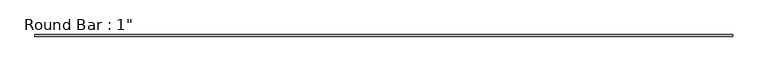
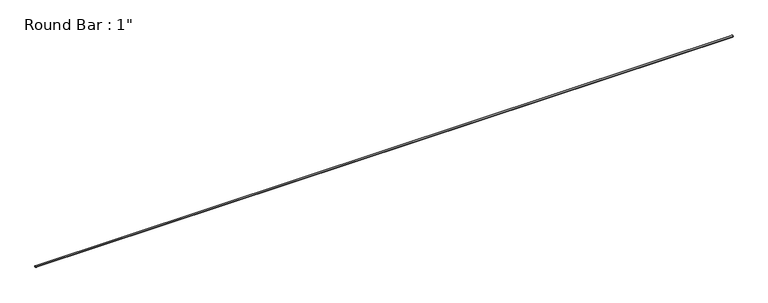
"""IFC4 building model written with IfcOpenShell, lengths in millimetres: member geometry."""

from ifc_helpers import new_model, si_unit, point, frame, origin, origin_2d, place, context, project, spatial, circle_curve, trimmed, segment, composite_curve, outline, extrude, source, transform, mapped, element, save


def member_a7b351ab(model_context):
    return source(origin(), model_context, "Body", "SweptSolid", [
        extrude(outline(composite_curve([segment(trimmed(circle_curve(origin_2d(), 12.7), [point((-12.7, 0.0))], [point((12.7, 0.0))], False, "CARTESIAN"), True, "CONTINUOUS"), segment(trimmed(circle_curve(origin_2d(), 12.7), [point((12.7, 0.0))], [point((-12.7, 0.0))], False, "CARTESIAN"), True, "CONTINUOUS")], self_intersect=False)), frame((-5486.4, 0.0, 0.0), z_axis=(1.0, 0.0, 0.0), x_axis=(0.0, 1.0, 0.0)), (0.0, 0.0, 1.0), 10972.8),
    ])


if __name__ == "__main__":
    model = new_model("IFC4")
    model_context = context("Model", 3, world=origin())
    ifc_project = project(units=[si_unit("LENGTHUNIT", "METRE", prefix="MILLI")], contexts=[model_context])
    site = spatial("IfcSite", under=ifc_project)
    building = spatial("IfcBuilding", under=site)
    placement = place(None, origin())
    member_shape = member_a7b351ab(model_context)
    element("IfcMember", 1, ObjectType="Round Bar : 1\"", at=placement, inside=building, context=model_context, shape_type="MappedRepresentation", body=[
        mapped(member_shape, transform((0.0, 0.0, 0.0), x_axis=(1.0, 0.0, 0.0), y_axis=(0.0, 1.0, 0.0), z_axis=(0.0, 0.0, 1.0))),
    ])
    save(model, "model.ifc")

# Revit data of these elements
# Type "Round Bar : 1\""
#   Assembly Code = "B10"
#   W = 0
#   Start Extension Calculation [instance default] = 10' - 0"
#   Start Extension [instance default] = -0' - 0 1/2"
#   End Extension Calculation [instance default] = 10' - 0"
#   End Extension [instance default] = -0' - 0 1/2"
#   Length [instance default] = 5' - 0"
#   d = 0' - 1"
#   A = 0 SF
#   Structural Material [instance default] = Metal - Steel - ASTM A36
# Element 1 (IfcMember, "Round Bar : 1\"")
#   Materials on its faces: "Metal - Steel - ASTM A36"
# Materials
#   "Metal - Steel - ASTM A36": class "Metal", colour RGB 199 199 199, transparency 0
